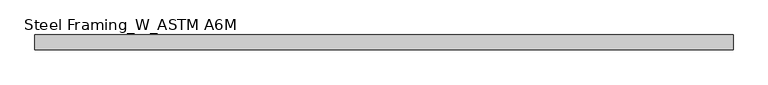
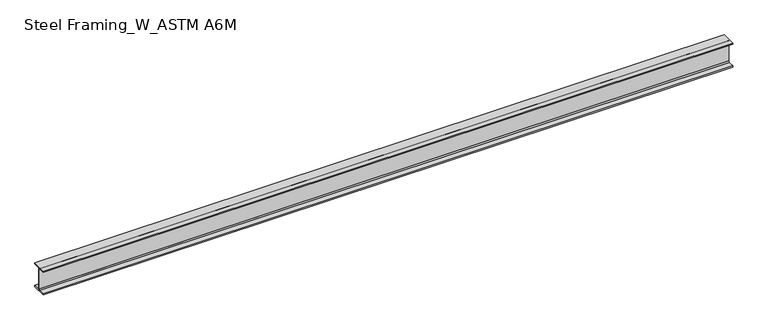
"""IFC4 building model written with IfcOpenShell, lengths in millimetres: beam geometry, Steel Framing_W_ASTM A6M : H_SB_AR_S02_W360x79_B2."""

from ifc_helpers import new_model, si_unit, point, frame, frame_2d, origin, place, context, project, spatial, polyline, circle_curve, trimmed, segment, composite_curve, outline, extrude, source, transform, mapped, element, save


def steel_framing_w_astm_a6m_d888c6d0(model_context):
    return source(origin(), model_context, "Body", "SweptSolid", [
        extrude(outline(composite_curve([segment(polyline([(102.5, -159.7), (102.5, -176.5), (-102.5, -176.5), (-102.5, -159.7), (-19.7, -159.7)]), True, "CONTINUOUS"), segment(trimmed(circle_curve(frame_2d((-19.7, -144.7)), 15.0), [point((-19.7, -159.7))], [point((-4.7, -144.7))], True, "CARTESIAN"), True, "CONTINUOUS"), segment(polyline([(-4.7, -144.7), (-4.7, 144.7)]), True, "CONTINUOUS"), segment(trimmed(circle_curve(frame_2d((-19.7, 144.7)), 15.0), [point((-4.7, 144.7))], [point((-19.7, 159.7))], True, "CARTESIAN"), True, "CONTINUOUS"), segment(polyline([(-19.7, 159.7), (-102.5, 159.7), (-102.5, 176.5), (102.5, 176.5), (102.5, 159.7), (19.7, 159.7)]), True, "CONTINUOUS"), segment(trimmed(circle_curve(frame_2d((19.7, 144.7)), 15.0), [point((19.7, 159.7))], [point((4.7, 144.7))], True, "CARTESIAN"), True, "CONTINUOUS"), segment(polyline([(4.7, 144.7), (4.7, -144.7)]), True, "CONTINUOUS"), segment(trimmed(circle_curve(frame_2d((19.7, -144.7)), 15.0), [point((4.7, -144.7))], [point((19.7, -159.7))], True, "CARTESIAN"), True, "CONTINUOUS"), segment(polyline([(19.7, -159.7), (102.5, -159.7)]), True, "CONTINUOUS")], self_intersect=False)), frame((-4846.3, 0.0, 0.0), z_axis=(1.0, 0.0, 0.0), x_axis=(0.0, 1.0, 0.0)), (0.0, 0.0, 1.0), 9692.6),
    ])


if __name__ == "__main__":
    model = new_model("IFC4")
    model_context = context("Model", 3, world=origin())
    ifc_project = project(units=[si_unit("LENGTHUNIT", "METRE", prefix="MILLI")], contexts=[model_context])
    site = spatial("IfcSite", under=ifc_project)
    building = spatial("IfcBuilding", under=site)
    placement = place(None, origin())
    steel_framing_w_astm_a6m_shape = steel_framing_w_astm_a6m_d888c6d0(model_context)
    element("IfcBeam", 1, ObjectType="Steel Framing_W_ASTM A6M : H_SB_AR_S02_W360x79_B2", at=placement, inside=building, context=model_context, shape_type="MappedRepresentation", body=[
        mapped(steel_framing_w_astm_a6m_shape, transform((0.0, 0.0, 0.0), x_axis=(1.0, 0.0, 0.0), y_axis=(0.0, 1.0, 0.0), z_axis=(0.0, 0.0, 1.0))),
    ])
    save(model, "model.ifc")

# Revit data of these elements
# Type "Steel Framing_W_ASTM A6M : H_SB_AR_S02_W360x79_B2"
#   Section Name Key = "W14x53"
#   Width = 20.5 cm
#   Web Thickness = 0.94 cm
#   Web Fillet = 1.5 cm
#   Warping Constant = 682000.0 cm⁶
#   Torsional Moment of Inertia = 80.70 cm⁴
#   Section Area = 101.0 cm²
#   Plastic Modulus weak axis = 361.0 cm³
#   Plastic Modulus strong axis = 1430.0 cm³
#   Perimeter = 1.48 m²/m
#   Nominal Weight = 79.00 kgf/m
#   Moment of Inertia weak axis = 2400.00 cm⁴
#   Moment of Inertia strong axis = 22500.00 cm⁴
#   Height = 35.3 cm
#   Flange Thickness = 1.68 cm
#   Elastic Modulus weak axis = 234.0 cm³
#   Elastic Modulus strong axis = 1270.0 cm³
#   Centroid Vertical = 17.65 cm
#   Centroid Horizontal = 10.25 cm
#   Length [instance default] = 1500 mm
#   Structural Material [instance default] = Steel, 45-345
#   Bolt Spacing = 0
#   Assembly Code = ""
# Element 1 (IfcBeam, "Steel Framing_W_ASTM A6M : H_SB_AR_S02_W360x79_B2")
#   Materials on its faces: "Steel, 45-345"
# Materials
#   "Steel, 45-345": class "Metal", colour RGB 189 187 185, transparency 0, Description = "Steel 345 MPa", Cost = 0
